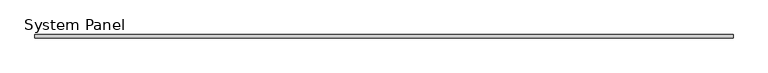
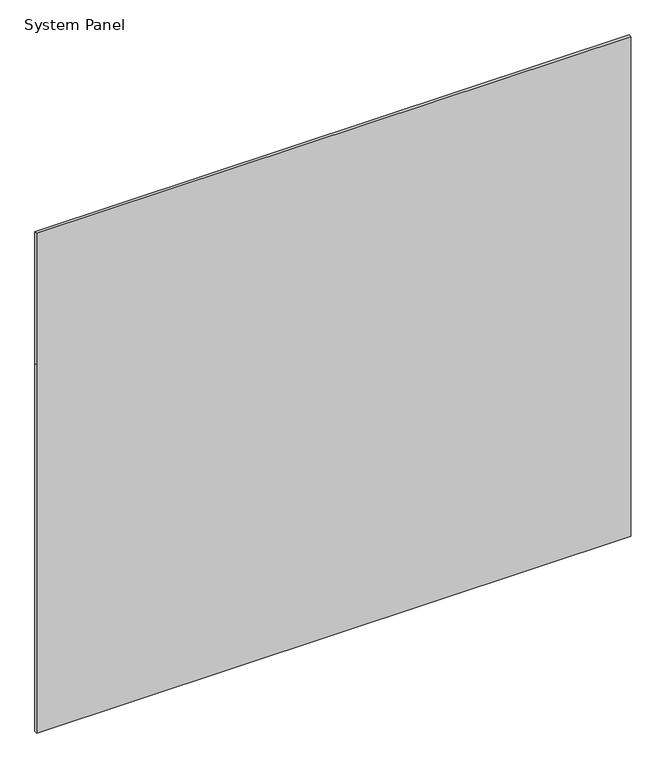
"""IFC4 building model written with IfcOpenShell, lengths in millimetres: plate geometry, System Panel : 로이복층유리_16."""

from ifc_helpers import new_model, si_unit, frame, origin, place, context, project, spatial, polyline, outline, extrude, source, transform, mapped, element, save


def system_panel_f4da12a8(model_context):
    return source(origin(), model_context, "Body", "SweptSolid", [
        extrude(outline(polyline([(0.0, -1662.5), (0.0, 1662.5), (2177.5, 1662.5), (2955.0, 1662.5), (2955.0, -1662.5), (2177.5, -1662.5), (0.0, -1662.5)])), frame((0.0, -8.0, 0.0), z_axis=(0.0, 1.0, 0.0), x_axis=(0.0, 0.0, 1.0)), (0.0, 0.0, 1.0), 16.0),
    ])


if __name__ == "__main__":
    model = new_model("IFC4")
    model_context = context("Model", 3, world=origin())
    ifc_project = project(units=[si_unit("LENGTHUNIT", "METRE", prefix="MILLI")], contexts=[model_context])
    site = spatial("IfcSite", under=ifc_project)
    building = spatial("IfcBuilding", under=site)
    placement = place(None, origin())
    system_panel_shape = system_panel_f4da12a8(model_context)
    element("IfcPlate", 1, ObjectType="System Panel : 로이복층유리_16", at=placement, inside=building, context=model_context, shape_type="MappedRepresentation", body=[
        mapped(system_panel_shape, transform((0.0, 0.0, 0.0), x_axis=(1.0, 0.0, 0.0), y_axis=(0.0, 1.0, 0.0), z_axis=(0.0, 0.0, 1.0))),
    ])
    save(model, "model.ifc")

# Revit data of these elements
# Element 1 (IfcPlate, "System Panel : 로이복층유리_16")
#   Materials on its faces: "00_Glass_Glass"
# Materials
#   "00_Glass_Glass": class "Glass", colour RGB 218 227 224, transparency 0.85, Description = "Glass", Cost = 0, Image = none
